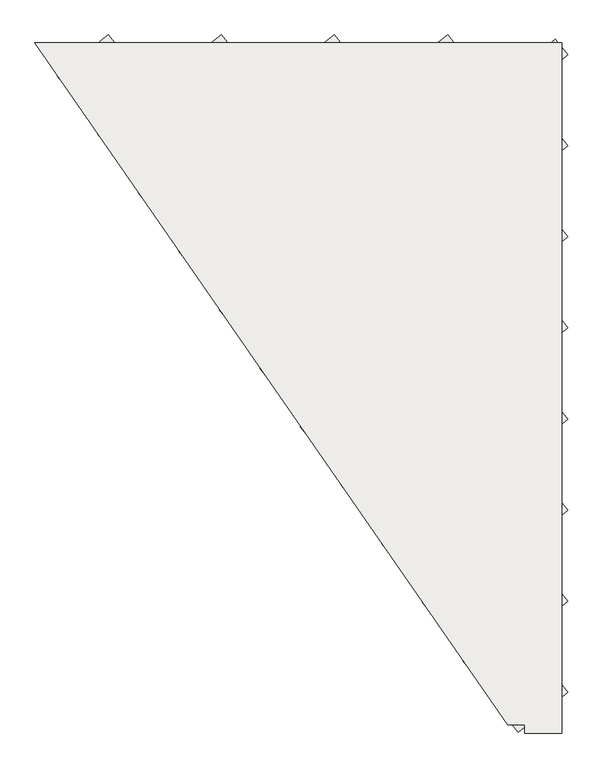
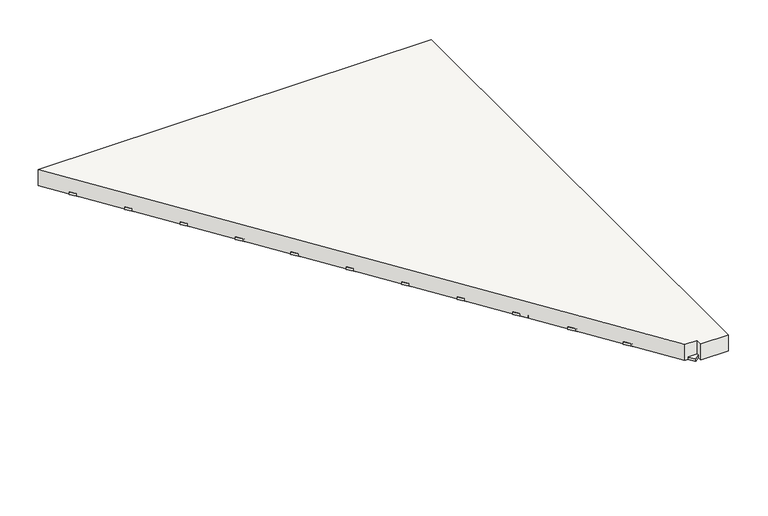
"""IFC4 building model written with IfcOpenShell, lengths in millimetres: slab geometry, Pano 14 (16 cm)."""

from ifc_helpers import new_model, si_unit, origin, origin_with_axes, place, context, project, spatial, polyline, outline, extrude, source, transform, mapped, element, save


def slab_2e18c83b(model_context):
    return source(origin(), model_context, "Body", "SweptSolid", [
        extrude(outline(polyline([(5948.237492, 10355.0), (9660.0, 10355.0), (9660.0, 5490.0), (9400.0, 5490.0), (9400.0, 5550.0), (9281.523496, 5550.0), (5948.237492, 10355.0)])), origin_with_axes(), (0.0, 0.0, 1.0), 160.0),
        extrude(outline(polyline([(7769.0309613, 9534.2272323), (7543.1786287, 9814.5676037), (7928.6466393, 10125.1145611), (8154.498972, 9844.7741898), (7769.0309613, 9534.2272323)])), origin_with_axes(), (0.0, 0.0, 1.0), 120.0),
        extrude(outline(polyline([(9050.2831684, 5892.1324632), (8962.4517056, 6001.1537188), (9616.0842689, 6527.7437294), (9703.9157317, 6418.7224739), (9050.2831684, 5892.1324632)])), origin_with_axes(), (0.0, 0.0, 1.0), 24.0),
        extrude(outline(polyline([(6764.4553744, 9187.2000132), (6676.6239116, 9296.2212688), (8058.5000632, 10409.5106276), (8146.3315259, 10300.4893721), (6764.4553744, 9187.2000132)])), origin_with_axes(), (0.0, 0.0, 1.0), 24.0),
        extrude(outline(polyline([(7050.1838484, 8775.3165692), (6962.3523856, 8884.3378248), (8855.480984, 10409.5106278), (8943.3124467, 10300.4893723), (7050.1838484, 8775.3165692)])), origin_with_axes(), (0.0, 0.0, 1.0), 24.0),
        extrude(outline(polyline([(6704.5792333, 9318.7430853), (6478.7269007, 9599.0834567), (6864.1949113, 9909.6304141), (7090.047244, 9629.2900428), (6704.5792333, 9318.7430853)])), origin_with_axes(), (0.0, 0.0, 1.0), 120.0),
        extrude(outline(polyline([(6192.9984264, 10010.9669022), (6105.1669636, 10119.9881578), (6464.5382227, 10409.5106292), (6552.3696854, 10300.4893737), (6192.9984264, 10010.9669022)])), origin_with_axes(), (0.0, 0.0, 1.0), 24.0),
        extrude(outline(polyline([(7847.4931293, 7671.2093103), (7621.6407967, 7951.5496817), (8007.1088073, 8262.0966391), (8232.96114, 7981.7562678), (7847.4931293, 7671.2093103)])), origin_with_axes(), (0.0, 0.0, 1.0), 120.0),
        extrude(outline(polyline([(8704.6785523, 6435.5589793), (8478.8262197, 6715.8993507), (8864.2942303, 7026.4463081), (9090.146563, 6746.1059368), (8704.6785523, 6435.5589793)])), origin_with_axes(), (0.0, 0.0, 1.0), 120.0),
        extrude(outline(polyline([(7483.3024873, 9946.1106743), (7257.4501547, 10226.4510457), (7345.45699, 10297.3525322), (7571.3093227, 10017.0121608), (7483.3024873, 9946.1106743)])), origin_with_axes(), (0.0, 0.0, 1.0), 120.0),
        extrude(outline(polyline([(8764.5546934, 6304.0159072), (8676.7232306, 6413.0371628), (9616.0842685, 7169.8203567), (9703.9157312, 7060.7991012), (8764.5546934, 6304.0159072)])), origin_with_axes(), (0.0, 0.0, 1.0), 24.0),
        extrude(outline(polyline([(9508.5727903, 9651.5117313), (9282.7204577, 9931.8521027), (9386.3383199, 10015.3303965), (9612.1906526, 9734.9900251), (9508.5727903, 9651.5117313)])), origin_with_axes(), (0.0, 0.0, 1.0), 120.0),
        extrude(outline(polyline([(7907.3692714, 7539.6662382), (7819.5378086, 7648.6874938), (9616.0842688, 9096.0502365), (9703.9157315, 8987.028981), (7907.3692714, 7539.6662382)])), origin_with_axes(), (0.0, 0.0, 1.0), 24.0),
        extrude(outline(polyline([(9119.2111633, 9337.8279363), (8893.3588307, 9618.1683077), (9278.8268413, 9928.7152651), (9504.679174, 9648.3748938), (9119.2111633, 9337.8279363)])), origin_with_axes(), (0.0, 0.0, 1.0), 120.0),
        extrude(outline(polyline([(9094.0401793, 6749.2427743), (8868.1878467, 7029.5831457), (9253.6558573, 7340.1301031), (9479.50819, 7059.7897318), (9094.0401793, 6749.2427743)])), origin_with_axes(), (0.0, 0.0, 1.0), 120.0),
        extrude(outline(polyline([(7621.6407974, 7951.5496822), (7533.8093346, 8060.5709378), (9616.0842692, 9738.1268637), (9703.9157319, 9629.1056081), (7621.6407974, 7951.5496822)])), origin_with_axes(), (0.0, 0.0, 1.0), 24.0),
        extrude(outline(polyline([(7093.9408603, 9632.4268813), (6868.0885277, 9912.7672527), (7253.5565383, 10223.3142101), (7479.408871, 9942.9738388), (7093.9408603, 9632.4268813)])), origin_with_axes(), (0.0, 0.0, 1.0), 120.0),
        extrude(outline(polyline([(9015.5780103, 8612.2606963), (8789.7256777, 8892.6010677), (9175.1936883, 9203.1480251), (9401.046021, 8922.8076538), (9015.5780103, 8612.2606963)])), origin_with_axes(), (0.0, 0.0, 1.0), 120.0),
        extrude(outline(polyline([(8444.1210623, 9436.0275843), (8218.2687297, 9716.3679557), (8603.7367403, 10026.9149131), (8829.589073, 9746.5745418), (8444.1210623, 9436.0275843)])), origin_with_axes(), (0.0, 0.0, 1.0), 120.0),
        extrude(outline(polyline([(7379.6693343, 9220.5434373), (7153.8170017, 9500.8838087), (7539.2850123, 9811.4307661), (7765.137345, 9531.0903948), (7379.6693343, 9220.5434373)])), origin_with_axes(), (0.0, 0.0, 1.0), 120.0),
        extrude(outline(polyline([(8418.9500783, 6847.4424233), (8193.0977457, 7127.7827947), (8578.5657563, 7438.3297521), (8804.418089, 7157.9893808), (8418.9500783, 6847.4424233)])), origin_with_axes(), (0.0, 0.0, 1.0), 120.0),
        extrude(outline(polyline([(8990.4070263, 6023.6755353), (8764.5546937, 6304.0159067), (9150.0227043, 6614.5628641), (9375.875037, 6334.2224928), (8990.4070263, 6023.6755353)])), origin_with_axes(), (0.0, 0.0, 1.0), 120.0),
        extrude(outline(polyline([(9197.6733323, 7474.8100133), (8971.8209997, 7755.1503847), (9357.2890103, 8065.6973421), (9583.141343, 7785.3569708), (9197.6733323, 7474.8100133)])), origin_with_axes(), (0.0, 0.0, 1.0), 120.0),
        extrude(outline(polyline([(8729.8495363, 9024.1441403), (8503.9972037, 9304.4845117), (8889.4652143, 9615.0314691), (9115.317547, 9334.6910978), (8729.8495363, 9024.1441403)])), origin_with_axes(), (0.0, 0.0, 1.0), 120.0),
        extrude(outline(polyline([(8340.4879093, 8710.4603453), (8114.6355767, 8990.8007167), (8500.1035873, 9301.3476741), (8725.95592, 9021.0073028), (8340.4879093, 8710.4603453)])), origin_with_axes(), (0.0, 0.0, 1.0), 120.0),
        extrude(outline(polyline([(8133.2216043, 7259.3258663), (7907.3692717, 7539.6662377), (8292.8372823, 7850.2131951), (8518.689615, 7569.8728238), (8133.2216043, 7259.3258663)])), origin_with_axes(), (0.0, 0.0, 1.0), 120.0),
        extrude(outline(polyline([(7335.9123234, 8363.4331252), (7248.0808606, 8472.4543808), (9616.0842688, 10380.2034892), (9703.9157315, 10271.1822337), (7335.9123234, 8363.4331252)])), origin_with_axes(), (0.0, 0.0, 1.0), 24.0),
        extrude(outline(polyline([(8193.0977454, 7127.7827942), (8105.2662826, 7236.8040498), (9616.0842684, 8453.9736094), (9703.9157311, 8344.9523538), (8193.0977454, 7127.7827942)])), origin_with_axes(), (0.0, 0.0, 1.0), 24.0),
        extrude(outline(polyline([(7665.3978083, 8808.6599933), (7439.5454757, 9089.0003647), (7825.0134863, 9399.5473221), (8050.865819, 9119.2069508), (7665.3978083, 8808.6599933)])), origin_with_axes(), (0.0, 0.0, 1.0), 120.0),
        extrude(outline(polyline([(8158.3925883, 9847.9110283), (7932.5402557, 10128.2513997), (8142.4379104, 10297.3525346), (8368.2902431, 10017.0121632), (8158.3925883, 9847.9110283)])), origin_with_axes(), (0.0, 0.0, 1.0), 120.0),
        extrude(outline(polyline([(9354.9288094, 5495.4893722), (9267.0973466, 5604.5106278), (9616.0842691, 5885.6671024), (9703.9157318, 5776.6458469), (9354.9288094, 5495.4893722)])), origin_with_axes(), (0.0, 0.0, 1.0), 24.0),
        extrude(outline(polyline([(6990.3077073, 8906.8596423), (6764.4553747, 9187.2000137), (7149.9233853, 9497.7469711), (7375.775718, 9217.4065998), (6990.3077073, 8906.8596423)])), origin_with_axes(), (0.0, 0.0, 1.0), 120.0),
        extrude(outline(polyline([(7561.7646553, 8083.0927543), (7335.9123227, 8363.4331257), (7721.3803333, 8673.9800831), (7947.232666, 8393.6397118), (7561.7646553, 8083.0927543)])), origin_with_axes(), (0.0, 0.0, 1.0), 120.0),
        extrude(outline(polyline([(8522.5832313, 7573.0096623), (8296.7308987, 7853.3500337), (8682.1989093, 8163.8969911), (8908.051242, 7883.5566198), (8522.5832313, 7573.0096623)])), origin_with_axes(), (0.0, 0.0, 1.0), 120.0),
        extrude(outline(polyline([(7951.1262823, 8396.7765493), (7725.2739497, 8677.1169207), (8110.7419603, 8987.6638781), (8336.594293, 8707.3235068), (7951.1262823, 8396.7765493)])), origin_with_axes(), (0.0, 0.0, 1.0), 120.0),
        extrude(outline(polyline([(9301.3064843, 8200.3772533), (9075.4541517, 8480.7176247), (9386.3383193, 8731.1771433), (9612.190652, 8450.8367719), (9301.3064843, 8200.3772533)])), origin_with_axes(), (0.0, 0.0, 1.0), 120.0),
        extrude(outline(polyline([(8833.4826893, 9749.7113793), (8607.6303567, 10030.0517507), (8939.4188308, 10297.352534), (9165.2711635, 10017.0121626), (8833.4826893, 9749.7113793)])), origin_with_axes(), (0.0, 0.0, 1.0), 120.0),
        extrude(outline(polyline([(8911.9448573, 7886.6934573), (8686.0925247, 8167.0338287), (9071.5605353, 8477.5807861), (9297.412868, 8197.2404148), (8911.9448573, 7886.6934573)])), origin_with_axes(), (0.0, 0.0, 1.0), 120.0),
        extrude(outline(polyline([(9483.4018063, 7062.9265703), (9257.5494737, 7343.2669417), (9386.0388105, 7446.7825942), (9611.8911432, 7166.4422228), (9483.4018063, 7062.9265703)])), origin_with_axes(), (0.0, 0.0, 1.0), 120.0),
        extrude(outline(polyline([(8054.7594353, 9122.3437893), (7828.9071027, 9402.6841607), (8214.3751133, 9713.2311181), (8440.227446, 9432.8907468), (8054.7594353, 9122.3437893)])), origin_with_axes(), (0.0, 0.0, 1.0), 120.0),
        extrude(outline(polyline([(8236.8547563, 7984.8931063), (8011.0024237, 8265.2334777), (8396.4704343, 8575.7804351), (8622.322767, 8295.4400638), (8236.8547563, 7984.8931063)])), origin_with_axes(), (0.0, 0.0, 1.0), 120.0),
        extrude(outline(polyline([(6478.7269004, 9599.0834572), (6390.8954376, 9708.1047128), (7261.5191431, 10409.5106281), (7349.3506058, 10300.4893725), (6478.7269004, 9599.0834572)])), origin_with_axes(), (0.0, 0.0, 1.0), 24.0),
        extrude(outline(polyline([(9379.7686533, 6337.3593303), (9153.9163207, 6617.6997017), (9386.3383196, 6804.9472621), (9612.1906523, 6524.6068907), (9379.7686533, 6337.3593303)])), origin_with_axes(), (0.0, 0.0, 1.0), 120.0),
        extrude(outline(polyline([(8808.3117053, 7161.1262183), (8582.4593727, 7441.4665897), (8967.9273833, 7752.0135471), (9193.779716, 7471.6731758), (8808.3117053, 7161.1262183)])), origin_with_axes(), (0.0, 0.0, 1.0), 120.0),
        extrude(outline(polyline([(8626.2163833, 8298.5769013), (8400.3640507, 8578.9172727), (8785.8320613, 8889.4642301), (9011.684394, 8609.1238588), (8626.2163833, 8298.5769013)])), origin_with_axes(), (0.0, 0.0, 1.0), 120.0),
        extrude(outline(polyline([(9404.9396373, 8925.9444923), (9179.0873047, 9206.2848637), (9386.3383196, 9373.2537699), (9612.1906523, 9092.9133985), (9404.9396373, 8925.9444923)])), origin_with_axes(), (0.0, 0.0, 1.0), 120.0),
        extrude(outline(polyline([(8478.8262194, 6715.8993502), (8390.9947566, 6824.9206058), (9616.0842681, 7811.8969822), (9703.9157308, 7702.8757267), (8478.8262194, 6715.8993502)])), origin_with_axes(), (0.0, 0.0, 1.0), 24.0),
        extrude(outline(polyline([(9587.0349593, 7788.4938093), (9361.1826267, 8068.8341807), (9386.3383201, 8089.1005163), (9612.1906528, 7808.7601449), (9587.0349593, 7788.4938093)])), origin_with_axes(), (0.0, 0.0, 1.0), 120.0),
        extrude(outline(polyline([(7276.0361813, 8494.9761983), (7050.1838487, 8775.3165697), (7435.6518593, 9085.8635271), (7661.504192, 8805.5231558), (7276.0361813, 8494.9761983)])), origin_with_axes(), (0.0, 0.0, 1.0), 120.0),
    ])


if __name__ == "__main__":
    model = new_model("IFC4")
    model_context = context("Model", 3, world=origin())
    ifc_project = project(units=[si_unit("LENGTHUNIT", "METRE", prefix="MILLI")], contexts=[model_context])
    site = spatial("IfcSite", under=ifc_project)
    building = spatial("IfcBuilding", under=site)
    placement = place(None, origin())
    slab_shape = slab_2e18c83b(model_context)
    element("IfcSlab", 1, ObjectType="Pano 14 (16 cm)", at=placement, inside=building, context=model_context, shape_type="MappedRepresentation", body=[
        mapped(slab_shape, transform((0.0, 0.0, 0.0), x_axis=(1.0, 0.0, 0.0), y_axis=(0.0, 1.0, 0.0), z_axis=(0.0, 0.0, 1.0))),
    ])
    save(model, "model.ifc")

# Revit data of these elements
# Element 1 (IfcSlab, "Pano 14 (16 cm)")
#   Materials on its faces: "Molde de poliestireno", "Concreto armado", "RGB 168-169-158"
# Materials
#   "Molde de poliestireno": class "Não atribuído", colour RGB 255 255 255, transparency 0
#   "Concreto armado": class "Não atribuído", colour RGB 168 169 158, transparency 0
#   "RGB 168-169-158": class "Não atribuído", colour RGB 168 169 158, transparency 0
